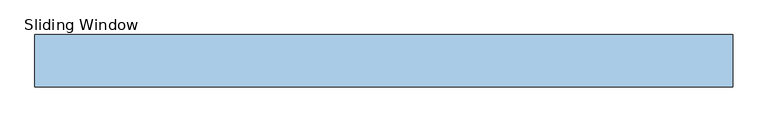
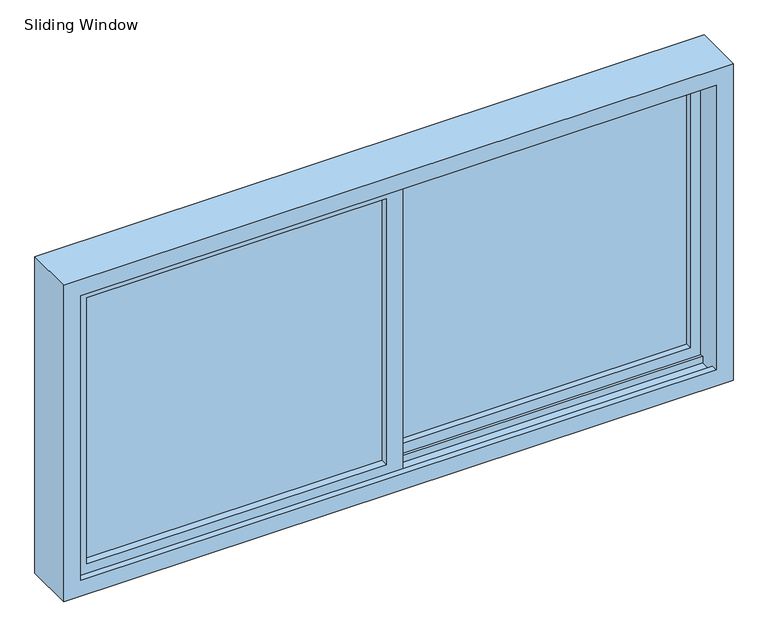
"""IFC4 building model written with IfcOpenShell, lengths in millimetres: window geometry, Sliding Window : H_WD_AMB_Sliding_Steel Window_DG_W2000xH1000."""

import ifcopenshell
import ifcopenshell.guid

model = None  # the IFC model being written
_history = None  # IfcOwnerHistory: only IFC2X3 demands one
_inside = {}  # id of a spatial element -> (the spatial element, [elements in it])
_under = {}  # id of a project, library or spatial element -> (it, [spatial elements below it])
_declared = {}  # id of a project -> (the project, [libraries it declares])
_typed = {}  # id of a type object -> (the type object, [elements of that type])
_made_of = {}  # id of a material, layer set ... -> (it, [elements and type objects made of it])


def new_model(schema):
    """Start an empty IFC model of exactly this schema.

    Asked for "IFC4X3", IfcOpenShell would pick the latest addendum, in which some entities
    have other attributes; the version numbers below select the first issue.
    IFC2X3 requires an IfcOwnerHistory on every rooted entity: one is made here for all.
    """
    global model, _history
    if schema == "IFC4X3":
        model = ifcopenshell.file(schema_version=(4, 3, 0, 0))
    else:
        model = ifcopenshell.file(schema=schema)
    _inside.clear()
    _under.clear()
    _declared.clear()
    _typed.clear()
    _made_of.clear()
    _history = None
    if model.schema == "IFC2X3":
        org = make("IfcOrganization", Name="unknown")
        user = make(
            "IfcPersonAndOrganization",
            ThePerson=make("IfcPerson", FamilyName="unknown"),
            TheOrganization=org,
        )
        app = make(
            "IfcApplication",
            ApplicationDeveloper=org,
            Version="unknown",
            ApplicationFullName="unknown",
            ApplicationIdentifier="unknown",
        )
        _history = make(
            "IfcOwnerHistory",
            OwningUser=user,
            OwningApplication=app,
            ChangeAction="ADDED",
            CreationDate=0,
        )
    return model


def make(cls, **values):
    """One entity of the class cls with the attributes given. An attribute that is None is left unset."""
    return model.create_entity(
        cls, **{name: value for name, value in values.items() if value is not None}
    )


def rooted(cls, **values):
    """An entity with a GlobalId (a new one), such as an element, a storey or a relation."""
    return make(cls, GlobalId=ifcopenshell.guid.new(), OwnerHistory=_history, **values)


def si_unit(unit_type, name, prefix=None):
    """IfcSIUnit, for example si_unit("LENGTHUNIT", "METRE", prefix="MILLI")."""
    return make("IfcSIUnit", UnitType=unit_type, Prefix=prefix, Name=name)


def assignment(units):
    """IfcUnitAssignment: the units of a project."""
    return None if units is None else make("IfcUnitAssignment", Units=units)


def point(xyz):
    """IfcCartesianPoint."""
    return None if xyz is None else make("IfcCartesianPoint", Coordinates=xyz)


def direction(xyz):
    """IfcDirection."""
    return None if xyz is None else make("IfcDirection", DirectionRatios=xyz)


def frame(location, z_axis=None, x_axis=None):
    """IfcAxis2Placement3D, a coordinate frame: its origin and axes. An axis left out is left unset."""
    return make(
        "IfcAxis2Placement3D",
        Location=point(location),
        Axis=direction(z_axis),
        RefDirection=direction(x_axis),
    )


def origin():
    """The frame at (0, 0, 0) with its axes left unset."""
    return frame((0.0, 0.0, 0.0))


def place(relative_to, where):
    """IfcLocalPlacement: puts the frame where relative to a parent placement (None: the world)."""
    return make(
        "IfcLocalPlacement", PlacementRelTo=relative_to, RelativePlacement=where
    )


def context(
    kind, dimensions, precision=None, world=None, true_north=None, identifier=None
):
    """IfcGeometricRepresentationContext, for example the 3D "Model" context."""
    return make(
        "IfcGeometricRepresentationContext",
        ContextIdentifier=identifier,
        ContextType=kind,
        CoordinateSpaceDimension=dimensions,
        Precision=precision,
        WorldCoordinateSystem=world,
        TrueNorth=true_north,
    )


def project(units=None, contexts=None):
    """IfcProject with its units and contexts."""
    return rooted(
        "IfcProject",
        Name="project",
        RepresentationContexts=contexts,
        UnitsInContext=assignment(units),
    )


def spatial(cls, under=None, at=None, **own):
    """A site, building, storey or space (cls), placed at a placement, below another one or the project."""
    s = rooted(cls, ObjectPlacement=at, **own)
    if under is not None:
        _under.setdefault(under.id(), (under, []))[1].append(s)
    return s


def polyline(points):
    """IfcPolyline through the points."""
    return make("IfcPolyline", Points=[point(p) for p in points])


def outline(outer, holes=None, kind="AREA"):
    """IfcArbitraryClosedProfileDef: a profile drawn as a closed curve; with holes, ...WithVoids."""
    if holes is None:
        return make("IfcArbitraryClosedProfileDef", ProfileType=kind, OuterCurve=outer)
    return make(
        "IfcArbitraryProfileDefWithVoids",
        ProfileType=kind,
        OuterCurve=outer,
        InnerCurves=holes,
    )


def extrude(swept, where, along, depth):
    """IfcExtrudedAreaSolid: the profile swept, set in the frame where, extruded along a direction by depth."""
    return make(
        "IfcExtrudedAreaSolid",
        SweptArea=swept,
        Position=where,
        ExtrudedDirection=direction(along),
        Depth=depth,
    )


def faces_of(points, faces, orient=None, outer=None):
    """IfcFace entities. A face is a list of loops; a loop is a list of indices into points, from 0.

    orient and outer hold one flag for each loop. By default every Orientation is true, the
    first loop of a face is its IfcFaceOuterBound and the others are IfcFaceBound.
    """
    made = []
    for i, loops in enumerate(faces):
        bounds = []
        for j, loop in enumerate(loops):
            is_outer = j == 0 if outer is None else outer[i][j]
            bounds.append(
                make(
                    "IfcFaceOuterBound" if is_outer else "IfcFaceBound",
                    Bound=make("IfcPolyLoop", Polygon=[points[k] for k in loop]),
                    Orientation=True if orient is None else orient[i][j],
                )
            )
        made.append(make("IfcFace", Bounds=bounds))
    return made


def faceted_brep(points, faces, orient=None, outer=None, voids=None):
    """IfcFacetedBrep: a solid bounded by flat faces; with voids (closed shells), ...WithVoids."""
    shared = [point(p) for p in points]
    hull = make("IfcClosedShell", CfsFaces=faces_of(shared, faces, orient, outer))
    if voids is None:
        return make("IfcFacetedBrep", Outer=hull)
    return make(
        "IfcFacetedBrepWithVoids",
        Outer=hull,
        Voids=[
            make(cls, CfsFaces=faces_of(shared, fs, o, b)) for cls, fs, o, b in voids
        ],
    )


def shape(context_of_items, identifier, shape_type, items):
    """IfcShapeRepresentation: the items that make up one representation, for example the "Body"."""
    return make(
        "IfcShapeRepresentation",
        ContextOfItems=context_of_items,
        RepresentationIdentifier=identifier,
        RepresentationType=shape_type,
        Items=items,
    )


def source(mapping_origin, context_of_items, identifier, shape_type, items):
    """IfcRepresentationMap: a shape defined once, which mapped items show again and again."""
    return make(
        "IfcRepresentationMap",
        MappingOrigin=mapping_origin,
        MappedRepresentation=shape(context_of_items, identifier, shape_type, items),
    )


def transform(
    local_origin,
    x_axis=None,
    y_axis=None,
    z_axis=None,
    scale=None,
    scale2=None,
    scale3=None,
    uniform=True,
):
    """IfcCartesianTransformationOperator3D, or its non-uniform kind. x_axis, y_axis, z_axis: its Axis1, 2, 3."""
    if uniform:
        return make(
            "IfcCartesianTransformationOperator3D",
            Axis1=direction(x_axis),
            Axis2=direction(y_axis),
            LocalOrigin=point(local_origin),
            Scale=scale,
            Axis3=direction(z_axis),
        )
    return make(
        "IfcCartesianTransformationOperator3DnonUniform",
        Axis1=direction(x_axis),
        Axis2=direction(y_axis),
        LocalOrigin=point(local_origin),
        Scale=scale,
        Axis3=direction(z_axis),
        Scale2=scale2,
        Scale3=scale3,
    )


def mapped(mapping_source, mapping_target):
    """IfcMappedItem: shows the shape of a source again, moved by a transform."""
    return make(
        "IfcMappedItem", MappingSource=mapping_source, MappingTarget=mapping_target
    )


def made_of(thing, what):
    """Note that an element or type object is made of a material, layer set ...; save() writes the relation."""
    if what is not None:
        _made_of.setdefault(what.id(), (what, []))[1].append(thing)
    return thing


def element(
    cls,
    number,
    at=None,
    inside=None,
    cuts=None,
    type_object=None,
    material=None,
    context=None,
    identifier="Body",
    shape_type=None,
    held_by="IfcProductDefinitionShape",
    body=None,
    shapes=None,
    **own,
):
    """One element of the class cls, such as IfcWall. Its Tag is "e" and its number.

    at: its placement. inside: the storey or other place that contains it. cuts: it is an
    opening in that element (IfcRelVoidsElement). A single representation is given by context,
    identifier, shape_type and body (its items); several are given by shapes. held_by: the class
    of the entity that holds the representations. save() writes the other relations.
    """
    e = rooted(cls, Tag="e%d" % number, ObjectPlacement=at, **own)
    if body is not None:
        shapes = [shape(context, identifier, shape_type, body)]
    if shapes is not None:
        e.Representation = make(held_by, Representations=shapes)
    if inside is not None:
        _inside.setdefault(inside.id(), (inside, []))[1].append(e)
    if cuts is not None:
        rooted(
            "IfcRelVoidsElement", RelatingBuildingElement=cuts, RelatedOpeningElement=e
        )
    if type_object is not None:
        _typed.setdefault(type_object.id(), (type_object, []))[1].append(e)
    return made_of(e, material)


def aggregate(whole, parts):
    """IfcRelAggregates: a whole, such as a stair, and the parts it consists of."""
    return rooted("IfcRelAggregates", RelatingObject=whole, RelatedObjects=parts)


def save(model, path):
    """Write the relations noted so far, then the file.

    IfcRelAggregates (storeys below a building ...), IfcRelContainedInSpatialStructure (elements
    in a storey), IfcRelDefinesByType, IfcRelAssociatesMaterial and IfcRelDeclares: one each for
    every whole, place, type object, material and project.
    """
    for whole, parts in _under.values():
        aggregate(whole, parts)
    for where, things in _inside.values():
        rooted(
            "IfcRelContainedInSpatialStructure",
            RelatedElements=things,
            RelatingStructure=where,
        )
    for kind, things in _typed.values():
        rooted("IfcRelDefinesByType", RelatedObjects=things, RelatingType=kind)
    for what, things in _made_of.values():
        rooted("IfcRelAssociatesMaterial", RelatedObjects=things, RelatingMaterial=what)
    for by, libraries in _declared.values():
        rooted("IfcRelDeclares", RelatingContext=by, RelatedDefinitions=libraries)
    model.write(path)


def sliding_window_5e64f0fd(model_context):
    return source(origin(), model_context, "Body", "SolidModel", [
        extrude(outline(polyline([(920.0, 27.5), (25.0, 27.5), (25.0, 32.5), (920.0, 32.5), (920.0, 27.5)])), frame((0.0, 0.0, 680.0), z_axis=(0.0, 0.0, 1.0), x_axis=(1.0, 0.0, 0.0)), (0.0, 0.0, 1.0), 840.0),
        extrude(outline(polyline([(-25.0, -32.5), (-920.0, -32.5), (-920.0, -27.5), (-25.0, -27.5), (-25.0, -32.5)])), frame((0.0, 0.0, 680.0), z_axis=(0.0, 0.0, 1.0), x_axis=(1.0, 0.0, 0.0)), (0.0, 0.0, 1.0), 840.0),
        extrude(outline(polyline([(630.0, -970.0), (630.0, 25.0), (1570.0, 25.0), (1570.0, -970.0), (630.0, -970.0)]), holes=[polyline([(1520.0, -920.0), (1520.0, -25.0), (680.0, -25.0), (680.0, -920.0), (1520.0, -920.0)])]), frame((0.0, -55.0, 0.0), z_axis=(0.0, 1.0, 0.0), x_axis=(0.0, 0.0, 1.0)), (0.0, 0.0, 1.0), 47.5),
        extrude(outline(polyline([(630.0, -25.0), (630.0, 970.0), (1570.0, 970.0), (1570.0, -25.0), (630.0, -25.0)]), holes=[polyline([(1520.0, 25.0), (1520.0, 920.0), (680.0, 920.0), (680.0, 25.0), (1520.0, 25.0)])]), frame((0.0, 7.5, 0.0), z_axis=(0.0, 1.0, 0.0), x_axis=(0.0, 0.0, 1.0)), (0.0, 0.0, 1.0), 45.0),
        faceted_brep([(-1000.0, 75.0, 1600.0), (-1000.0, 75.0, 600.0), (-1000.0, -75.0, 600.0), (-1000.0, -75.0, 1600.0), (1000.0, 75.0, 1600.0), (1000.0, 75.0, 600.0), (950.0, 75.0, 650.0), (950.0, 75.0, 1550.0), (-950.0, 75.0, 1550.0), (-950.0, 75.0, 650.0), (1000.0, -75.0, 600.0), (1000.0, -75.0, 1600.0), (-950.0, -75.0, 1550.0), (950.0, -75.0, 1550.0), (950.0, -75.0, 650.0), (-950.0, -75.0, 650.0), (950.0, 55.0, 650.0), (950.0, 55.0, 1550.0), (-950.0, 55.0, 1550.0), (-950.0, 55.0, 1570.0), (-950.0, 5.0, 1570.0), (-950.0, 5.0, 1550.0), (-950.0, -5.0, 1550.0), (-950.0, -5.0, 650.0), (-950.0, 5.0, 650.0), (-950.0, 5.0, 630.0), (-950.0, 55.0, 630.0), (-950.0, 55.0, 650.0), (950.0, -5.0, 650.0), (950.0, 5.0, 650.0), (950.0, -5.0, 630.0), (950.0, -55.0, 630.0), (950.0, -55.0, 650.0), (950.0, -55.0, 1550.0), (950.0, -55.0, 1570.0), (950.0, -5.0, 1570.0), (950.0, -5.0, 1550.0), (950.0, 5.0, 1550.0), (970.0, 5.0, 1570.0), (970.0, 5.0, 630.0), (-970.0, -5.0, 1570.0), (-970.0, -5.0, 630.0), (970.0, 55.0, 1570.0), (970.0, 55.0, 630.0), (-970.0, -55.0, 630.0), (-950.0, -55.0, 1550.0), (-950.0, -55.0, 650.0), (-970.0, -55.0, 1570.0)], [[[0, 1, 2, 3]], [[4, 5, 1, 0], [6, 7, 8, 9]], [[1, 5, 10, 2]], [[10, 11, 3, 2], [12, 13, 14, 15]], [[7, 6, 16, 17]], [[9, 8, 18, 19, 20, 21, 22, 23, 24, 25, 26, 27]], [[16, 6, 9, 27]], [[5, 4, 11, 10]], [[28, 29, 24, 23]], [[28, 30, 31, 32, 14, 13, 33, 34, 35, 36, 37, 29]], [[29, 37, 21, 20, 38, 39, 25, 24]], [[40, 41, 30, 28, 23, 22, 36, 35]], [[39, 38, 42, 43]], [[39, 43, 26, 25]], [[43, 42, 19, 18, 17, 16, 27, 26]], [[41, 44, 31, 30]], [[45, 46, 32, 31, 44, 47, 34, 33]], [[46, 15, 14, 32]], [[12, 15, 46, 45]], [[47, 44, 41, 40]], [[3, 11, 4, 0]], [[7, 17, 18, 8]], [[37, 36, 22, 21]], [[42, 38, 20, 19]], [[12, 45, 33, 13]], [[47, 40, 35, 34]]]),
    ])


if __name__ == "__main__":
    model = new_model("IFC4")
    model_context = context("Model", 3, world=origin())
    ifc_project = project(units=[si_unit("LENGTHUNIT", "METRE", prefix="MILLI")], contexts=[model_context])
    site = spatial("IfcSite", under=ifc_project)
    building = spatial("IfcBuilding", under=site)
    placement = place(None, origin())
    sliding_window_shape = sliding_window_5e64f0fd(model_context)
    element("IfcWindow", 1, ObjectType="Sliding Window : H_WD_AMB_Sliding_Steel Window_DG_W2000xH1000", at=placement, inside=building, context=model_context, shape_type="MappedRepresentation", body=[
        mapped(sliding_window_shape, transform((0.0, 0.0, 0.0), x_axis=(1.0, 0.0, 0.0), y_axis=(0.0, 1.0, 0.0), z_axis=(0.0, 0.0, 1.0))),
    ])
    save(model, "model.ifc")

# Revit data of these elements
# Project information
#   Building Name = "SULFUR LOADING CONTROL BD"
#   Project Status = "Project Status"
#   Client Name = "현대엔지니어링"
#   Project Address = "서울시 종로구 율곡로 75(계동)"
#   Project Number = "-"
# Type "Sliding Window : H_WD_AMB_Sliding_Steel Window_DG_W2000xH1000"
#   Description = "Steel Frame + 2 x T=6mm + T12mm Air Space"
#   Type Mark = ""
#   Analytic Construction = "<None>"
#   창 두께 = 150.000 mm
#   Visual Light Transmittance = 0.88
#   Thermal Resistance (R) = 0.271106 (m²·K)/W
#   Solar Heat Gain Coefficient = 0.81
#   Height = 1000.000 mm
#   Heat Transfer Coefficient (U) = 6.2426 W/(m²·K)
#   기본 씰 높이 = 600.000 mm
#   Width = 2000.000 mm
#   Define Thermal Properties by = 1
#   창 패널 = none
#   창 프레임 = none
#   Construction Type Id = ""
#   Wall Closure = (empty or 0)
